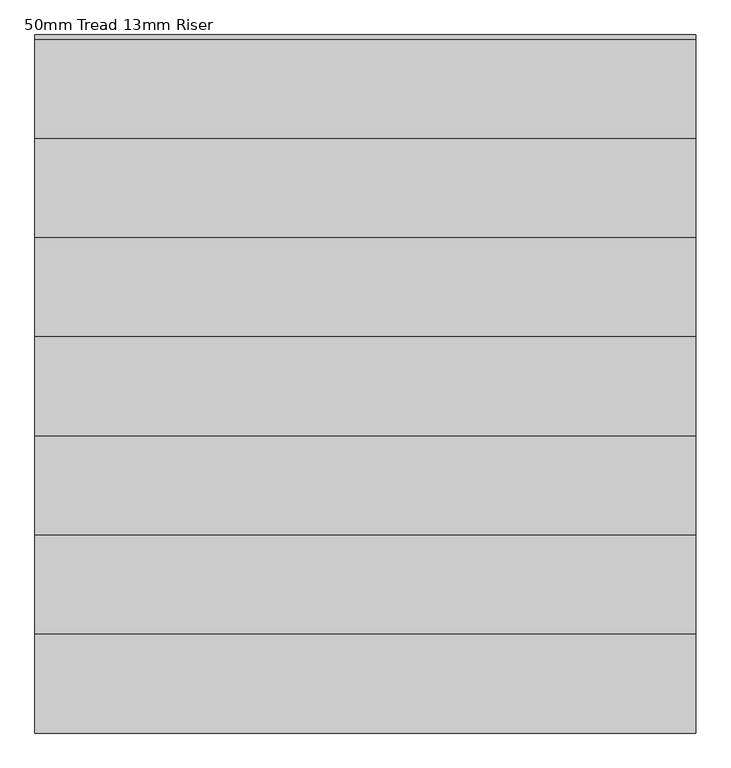
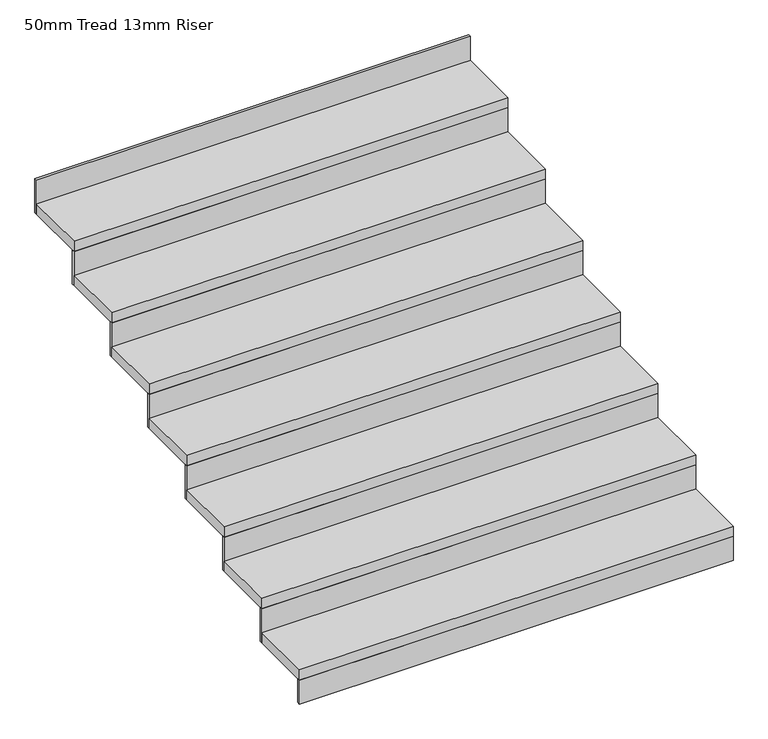
"""IFC4 building model written with IfcOpenShell, lengths in millimetres: stair flight geometry, 50mm Tread 13mm Riser."""

from ifc_helpers import new_model, si_unit, frame, origin, place, context, project, spatial, polyline, outline, extrude, source, transform, mapped, element, save


def stair_flight_50mm_tread_13mm_riser_a217ff0d(model_context):
    return source(origin(), model_context, "Body", "SweptSolid", [
        extrude(outline(polyline([(14700.0002443, 21382.4999999), (14700.0002443, 21369.9999999), (12700.0002443, 21369.9999999), (12700.0002443, 21382.4999999), (14700.0002443, 21382.4999999)])), frame((0.0, 0.0, 21000.0), z_axis=(0.0, 0.0, 1.0), x_axis=(1.0, 0.0, 0.0)), (0.0, 0.0, 1.0), 116.6666667),
        extrude(outline(polyline([(12700.0002443, 21669.9999999), (14700.0002443, 21669.9999999), (14700.0002443, 21369.9999999), (12700.0002443, 21369.9999999), (12700.0002443, 21669.9999999)])), frame((0.0, 0.0, 21116.6666667), z_axis=(0.0, 0.0, 1.0), x_axis=(1.0, 0.0, 0.0)), (0.0, 0.0, 1.0), 50.0),
        extrude(outline(polyline([(14700.0002443, 21682.4999999), (14700.0002443, 21669.9999999), (12700.0002443, 21669.9999999), (12700.0002443, 21682.4999999), (14700.0002443, 21682.4999999)])), frame((0.0, 0.0, 21116.6666667), z_axis=(0.0, 0.0, 1.0), x_axis=(1.0, 0.0, 0.0)), (0.0, 0.0, 1.0), 166.6666667),
        extrude(outline(polyline([(12700.0002443, 21969.9999999), (14700.0002443, 21969.9999999), (14700.0002443, 21669.9999999), (12700.0002443, 21669.9999999), (12700.0002443, 21969.9999999)])), frame((0.0, 0.0, 21283.3333333), z_axis=(0.0, 0.0, 1.0), x_axis=(1.0, 0.0, 0.0)), (0.0, 0.0, 1.0), 50.0),
        extrude(outline(polyline([(14700.0002443, 21982.4999999), (14700.0002443, 21969.9999999), (12700.0002443, 21969.9999999), (12700.0002443, 21982.4999999), (14700.0002443, 21982.4999999)])), frame((0.0, 0.0, 21283.3333333), z_axis=(0.0, 0.0, 1.0), x_axis=(1.0, 0.0, 0.0)), (0.0, 0.0, 1.0), 166.6666667),
        extrude(outline(polyline([(12700.0002443, 22269.9999999), (14700.0002443, 22269.9999999), (14700.0002443, 21969.9999999), (12700.0002443, 21969.9999999), (12700.0002443, 22269.9999999)])), frame((0.0, 0.0, 21450.0), z_axis=(0.0, 0.0, 1.0), x_axis=(1.0, 0.0, 0.0)), (0.0, 0.0, 1.0), 50.0),
        extrude(outline(polyline([(14700.0002443, 22282.4999999), (14700.0002443, 22269.9999999), (12700.0002443, 22269.9999999), (12700.0002443, 22282.4999999), (14700.0002443, 22282.4999999)])), frame((0.0, 0.0, 21450.0), z_axis=(0.0, 0.0, 1.0), x_axis=(1.0, 0.0, 0.0)), (0.0, 0.0, 1.0), 166.6666667),
        extrude(outline(polyline([(12700.0002443, 22569.9999999), (14700.0002443, 22569.9999999), (14700.0002443, 22269.9999999), (12700.0002443, 22269.9999999), (12700.0002443, 22569.9999999)])), frame((0.0, 0.0, 21616.6666667), z_axis=(0.0, 0.0, 1.0), x_axis=(1.0, 0.0, 0.0)), (0.0, 0.0, 1.0), 50.0),
        extrude(outline(polyline([(14700.0002443, 22582.4999999), (14700.0002443, 22569.9999999), (12700.0002443, 22569.9999999), (12700.0002443, 22582.4999999), (14700.0002443, 22582.4999999)])), frame((0.0, 0.0, 21616.6666667), z_axis=(0.0, 0.0, 1.0), x_axis=(1.0, 0.0, 0.0)), (0.0, 0.0, 1.0), 166.6666667),
        extrude(outline(polyline([(12700.0002443, 22869.9999999), (14700.0002443, 22869.9999999), (14700.0002443, 22569.9999999), (12700.0002443, 22569.9999999), (12700.0002443, 22869.9999999)])), frame((0.0, 0.0, 21783.3333333), z_axis=(0.0, 0.0, 1.0), x_axis=(1.0, 0.0, 0.0)), (0.0, 0.0, 1.0), 50.0),
        extrude(outline(polyline([(14700.0002443, 22882.4999999), (14700.0002443, 22869.9999999), (12700.0002443, 22869.9999999), (12700.0002443, 22882.4999999), (14700.0002443, 22882.4999999)])), frame((0.0, 0.0, 21783.3333333), z_axis=(0.0, 0.0, 1.0), x_axis=(1.0, 0.0, 0.0)), (0.0, 0.0, 1.0), 166.6666667),
        extrude(outline(polyline([(12700.0002443, 23169.9999999), (14700.0002443, 23169.9999999), (14700.0002443, 22869.9999999), (12700.0002443, 22869.9999999), (12700.0002443, 23169.9999999)])), frame((0.0, 0.0, 21950.0), z_axis=(0.0, 0.0, 1.0), x_axis=(1.0, 0.0, 0.0)), (0.0, 0.0, 1.0), 50.0),
        extrude(outline(polyline([(14700.0002443, 23182.4999999), (14700.0002443, 23169.9999999), (12700.0002443, 23169.9999999), (12700.0002443, 23182.4999999), (14700.0002443, 23182.4999999)])), frame((0.0, 0.0, 21950.0), z_axis=(0.0, 0.0, 1.0), x_axis=(1.0, 0.0, 0.0)), (0.0, 0.0, 1.0), 166.6666667),
        extrude(outline(polyline([(14700.0002443, 23482.4999999), (14700.0002443, 23469.9999999), (12700.0002443, 23469.9999999), (12700.0002443, 23482.4999999), (14700.0002443, 23482.4999999)])), frame((0.0, 0.0, 22116.6666667), z_axis=(0.0, 0.0, 1.0), x_axis=(1.0, 0.0, 0.0)), (0.0, 0.0, 1.0), 166.6666667),
        extrude(outline(polyline([(12700.0002443, 23469.9999999), (14700.0002443, 23469.9999999), (14700.0002443, 23169.9999999), (12700.0002443, 23169.9999999), (12700.0002443, 23469.9999999)])), frame((0.0, 0.0, 22116.6666667), z_axis=(0.0, 0.0, 1.0), x_axis=(1.0, 0.0, 0.0)), (0.0, 0.0, 1.0), 50.0),
    ])


if __name__ == "__main__":
    model = new_model("IFC4")
    model_context = context("Model", 3, world=origin())
    ifc_project = project(units=[si_unit("LENGTHUNIT", "METRE", prefix="MILLI")], contexts=[model_context])
    site = spatial("IfcSite", under=ifc_project)
    building = spatial("IfcBuilding", under=site)
    placement = place(None, origin())
    stair_flight_50mm_tread_13mm_riser_shape = stair_flight_50mm_tread_13mm_riser_a217ff0d(model_context)
    element("IfcStairFlight", 1, ObjectType="50mm Tread 13mm Riser", at=placement, inside=building, context=model_context, shape_type="MappedRepresentation", body=[
        mapped(stair_flight_50mm_tread_13mm_riser_shape, transform((0.0, 0.0, 0.0), x_axis=(1.0, 0.0, 0.0), y_axis=(0.0, 1.0, 0.0), z_axis=(0.0, 0.0, 1.0))),
    ])
    save(model, "model.ifc")
